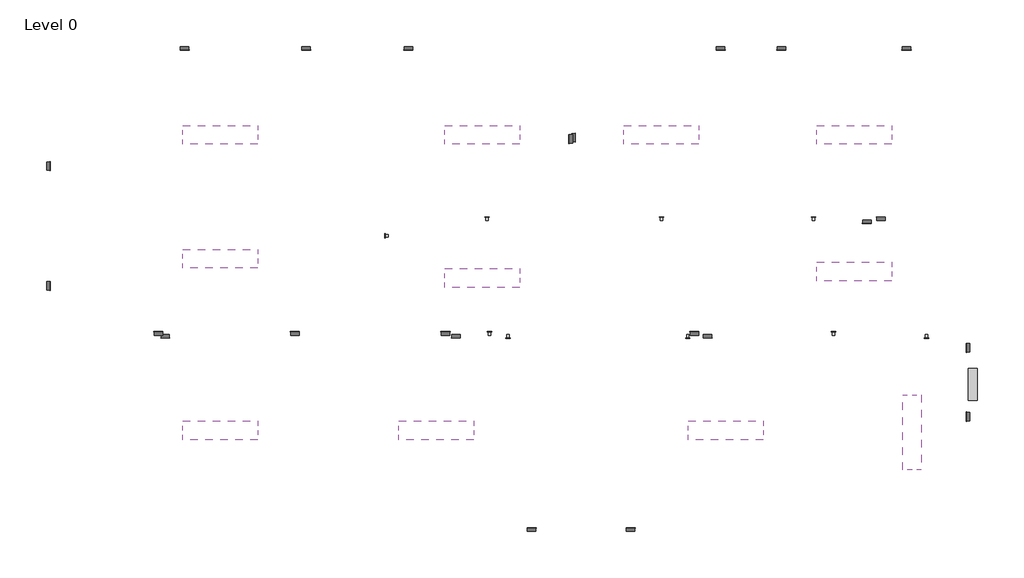
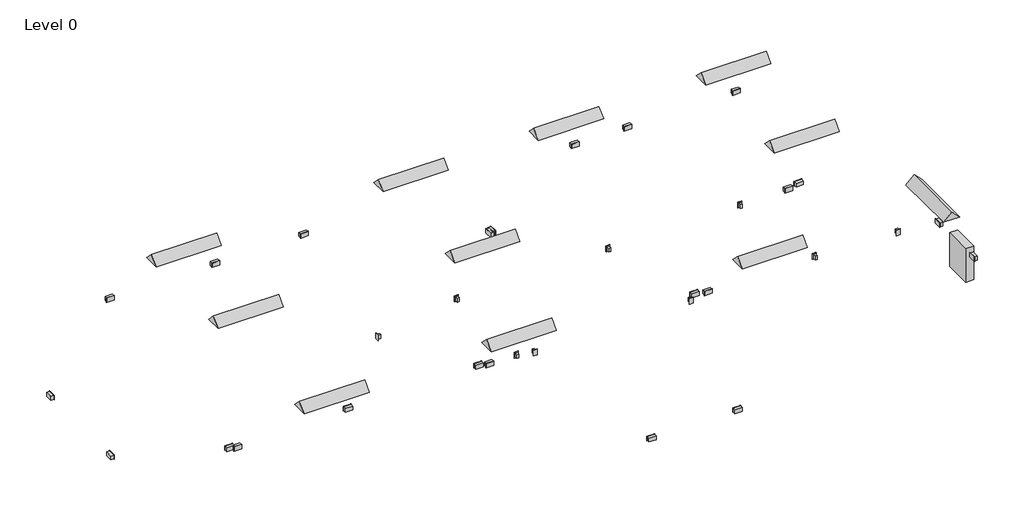
# One storey: 24 proxies, 11 light fixtures, 9 switching devices.
"""IFC4 building model written with IfcOpenShell, lengths in millimetres."""

import ifcopenshell
import ifcopenshell.guid

model = None  # the IFC model being written
_history = None  # IfcOwnerHistory: only IFC2X3 demands one
_inside = {}  # id of a spatial element -> (the spatial element, [elements in it])
_under = {}  # id of a project, library or spatial element -> (it, [spatial elements below it])
_declared = {}  # id of a project -> (the project, [libraries it declares])
_typed = {}  # id of a type object -> (the type object, [elements of that type])
_made_of = {}  # id of a material, layer set ... -> (it, [elements and type objects made of it])


def new_model(schema):
    """Start an empty IFC model of exactly this schema.

    Asked for "IFC4X3", IfcOpenShell would pick the latest addendum, in which some entities
    have other attributes; the version numbers below select the first issue.
    IFC2X3 requires an IfcOwnerHistory on every rooted entity: one is made here for all.
    """
    global model, _history
    if schema == "IFC4X3":
        model = ifcopenshell.file(schema_version=(4, 3, 0, 0))
    else:
        model = ifcopenshell.file(schema=schema)
    _inside.clear()
    _under.clear()
    _declared.clear()
    _typed.clear()
    _made_of.clear()
    _history = None
    if model.schema == "IFC2X3":
        org = make("IfcOrganization", Name="unknown")
        user = make(
            "IfcPersonAndOrganization",
            ThePerson=make("IfcPerson", FamilyName="unknown"),
            TheOrganization=org,
        )
        app = make(
            "IfcApplication",
            ApplicationDeveloper=org,
            Version="unknown",
            ApplicationFullName="unknown",
            ApplicationIdentifier="unknown",
        )
        _history = make(
            "IfcOwnerHistory",
            OwningUser=user,
            OwningApplication=app,
            ChangeAction="ADDED",
            CreationDate=0,
        )
    return model


def make(cls, **values):
    """One entity of the class cls with the attributes given. An attribute that is None is left unset."""
    return model.create_entity(
        cls, **{name: value for name, value in values.items() if value is not None}
    )


def rooted(cls, **values):
    """An entity with a GlobalId (a new one), such as an element, a storey or a relation."""
    return make(cls, GlobalId=ifcopenshell.guid.new(), OwnerHistory=_history, **values)


def si_unit(unit_type, name, prefix=None):
    """IfcSIUnit, for example si_unit("LENGTHUNIT", "METRE", prefix="MILLI")."""
    return make("IfcSIUnit", UnitType=unit_type, Prefix=prefix, Name=name)


def assignment(units):
    """IfcUnitAssignment: the units of a project."""
    return None if units is None else make("IfcUnitAssignment", Units=units)


def point(xyz):
    """IfcCartesianPoint."""
    return None if xyz is None else make("IfcCartesianPoint", Coordinates=xyz)


def direction(xyz):
    """IfcDirection."""
    return None if xyz is None else make("IfcDirection", DirectionRatios=xyz)


def frame(location, z_axis=None, x_axis=None):
    """IfcAxis2Placement3D, a coordinate frame: its origin and axes. An axis left out is left unset."""
    return make(
        "IfcAxis2Placement3D",
        Location=point(location),
        Axis=direction(z_axis),
        RefDirection=direction(x_axis),
    )


def origin():
    """The frame at (0, 0, 0) with its axes left unset."""
    return frame((0.0, 0.0, 0.0))


def origin_with_axes():
    """The frame at (0, 0, 0) with the z axis (0, 0, 1) and the x axis (1, 0, 0) written out."""
    return frame((0.0, 0.0, 0.0), z_axis=(0.0, 0.0, 1.0), x_axis=(1.0, 0.0, 0.0))


def place(relative_to, where):
    """IfcLocalPlacement: puts the frame where relative to a parent placement (None: the world)."""
    return make(
        "IfcLocalPlacement", PlacementRelTo=relative_to, RelativePlacement=where
    )


def context(
    kind, dimensions, precision=None, world=None, true_north=None, identifier=None
):
    """IfcGeometricRepresentationContext, for example the 3D "Model" context."""
    return make(
        "IfcGeometricRepresentationContext",
        ContextIdentifier=identifier,
        ContextType=kind,
        CoordinateSpaceDimension=dimensions,
        Precision=precision,
        WorldCoordinateSystem=world,
        TrueNorth=true_north,
    )


def project(units=None, contexts=None):
    """IfcProject with its units and contexts."""
    return rooted(
        "IfcProject",
        Name="project",
        RepresentationContexts=contexts,
        UnitsInContext=assignment(units),
    )


def spatial(cls, under=None, at=None, **own):
    """A site, building, storey or space (cls), placed at a placement, below another one or the project."""
    s = rooted(cls, ObjectPlacement=at, **own)
    if under is not None:
        _under.setdefault(under.id(), (under, []))[1].append(s)
    return s


def polyline(points):
    """IfcPolyline through the points."""
    return make("IfcPolyline", Points=[point(p) for p in points])


def outline(outer, holes=None, kind="AREA"):
    """IfcArbitraryClosedProfileDef: a profile drawn as a closed curve; with holes, ...WithVoids."""
    if holes is None:
        return make("IfcArbitraryClosedProfileDef", ProfileType=kind, OuterCurve=outer)
    return make(
        "IfcArbitraryProfileDefWithVoids",
        ProfileType=kind,
        OuterCurve=outer,
        InnerCurves=holes,
    )


def extrude(swept, where, along, depth):
    """IfcExtrudedAreaSolid: the profile swept, set in the frame where, extruded along a direction by depth."""
    return make(
        "IfcExtrudedAreaSolid",
        SweptArea=swept,
        Position=where,
        ExtrudedDirection=direction(along),
        Depth=depth,
    )


def shape(context_of_items, identifier, shape_type, items):
    """IfcShapeRepresentation: the items that make up one representation, for example the "Body"."""
    return make(
        "IfcShapeRepresentation",
        ContextOfItems=context_of_items,
        RepresentationIdentifier=identifier,
        RepresentationType=shape_type,
        Items=items,
    )


def source(mapping_origin, context_of_items, identifier, shape_type, items):
    """IfcRepresentationMap: a shape defined once, which mapped items show again and again."""
    return make(
        "IfcRepresentationMap",
        MappingOrigin=mapping_origin,
        MappedRepresentation=shape(context_of_items, identifier, shape_type, items),
    )


def transform(
    local_origin,
    x_axis=None,
    y_axis=None,
    z_axis=None,
    scale=None,
    scale2=None,
    scale3=None,
    uniform=True,
):
    """IfcCartesianTransformationOperator3D, or its non-uniform kind. x_axis, y_axis, z_axis: its Axis1, 2, 3."""
    if uniform:
        return make(
            "IfcCartesianTransformationOperator3D",
            Axis1=direction(x_axis),
            Axis2=direction(y_axis),
            LocalOrigin=point(local_origin),
            Scale=scale,
            Axis3=direction(z_axis),
        )
    return make(
        "IfcCartesianTransformationOperator3DnonUniform",
        Axis1=direction(x_axis),
        Axis2=direction(y_axis),
        LocalOrigin=point(local_origin),
        Scale=scale,
        Axis3=direction(z_axis),
        Scale2=scale2,
        Scale3=scale3,
    )


def mapped(mapping_source, mapping_target):
    """IfcMappedItem: shows the shape of a source again, moved by a transform."""
    return make(
        "IfcMappedItem", MappingSource=mapping_source, MappingTarget=mapping_target
    )


def made_of(thing, what):
    """Note that an element or type object is made of a material, layer set ...; save() writes the relation."""
    if what is not None:
        _made_of.setdefault(what.id(), (what, []))[1].append(thing)
    return thing


def element(
    cls,
    number,
    at=None,
    inside=None,
    cuts=None,
    type_object=None,
    material=None,
    context=None,
    identifier="Body",
    shape_type=None,
    held_by="IfcProductDefinitionShape",
    body=None,
    shapes=None,
    **own,
):
    """One element of the class cls, such as IfcWall. Its Tag is "e" and its number.

    at: its placement. inside: the storey or other place that contains it. cuts: it is an
    opening in that element (IfcRelVoidsElement). A single representation is given by context,
    identifier, shape_type and body (its items); several are given by shapes. held_by: the class
    of the entity that holds the representations. save() writes the other relations.
    """
    e = rooted(cls, Tag="e%d" % number, ObjectPlacement=at, **own)
    if body is not None:
        shapes = [shape(context, identifier, shape_type, body)]
    if shapes is not None:
        e.Representation = make(held_by, Representations=shapes)
    if inside is not None:
        _inside.setdefault(inside.id(), (inside, []))[1].append(e)
    if cuts is not None:
        rooted(
            "IfcRelVoidsElement", RelatingBuildingElement=cuts, RelatedOpeningElement=e
        )
    if type_object is not None:
        _typed.setdefault(type_object.id(), (type_object, []))[1].append(e)
    return made_of(e, material)


def aggregate(whole, parts):
    """IfcRelAggregates: a whole, such as a stair, and the parts it consists of."""
    return rooted("IfcRelAggregates", RelatingObject=whole, RelatedObjects=parts)


def save(model, path):
    """Write the relations noted so far, then the file.

    IfcRelAggregates (storeys below a building ...), IfcRelContainedInSpatialStructure (elements
    in a storey), IfcRelDefinesByType, IfcRelAssociatesMaterial and IfcRelDeclares: one each for
    every whole, place, type object, material and project.
    """
    for whole, parts in _under.values():
        aggregate(whole, parts)
    for where, things in _inside.values():
        rooted(
            "IfcRelContainedInSpatialStructure",
            RelatedElements=things,
            RelatingStructure=where,
        )
    for kind, things in _typed.values():
        rooted("IfcRelDefinesByType", RelatedObjects=things, RelatingType=kind)
    for what, things in _made_of.values():
        rooted("IfcRelAssociatesMaterial", RelatedObjects=things, RelatingMaterial=what)
    for by, libraries in _declared.values():
        rooted("IfcRelDeclares", RelatingContext=by, RelatedDefinitions=libraries)
    model.write(path)


def lighting_and_appliance_panelboard_400v_mlo_125_a_11cb7106(model_context):
    return source(origin(), model_context, "Body", "SweptSolid", [
        extrude(outline(polyline([(254.0, -660.4), (-254.0, -660.4), (-254.0, 0.0), (254.0, 0.0), (254.0, -660.4)])), frame((0.0, 0.0, -146.1), z_axis=(0.0, 0.0, 1.0), x_axis=(1.0, 0.0, 0.0)), (0.0, 0.0, 1.0), 146.1),
    ])


def twin_switched_socket_outlet_standard_0deee84c(model_context):
    return source(origin(), model_context, "Body", "SweptSolid", [
        extrude(outline(polyline([(67.5, 37.5), (67.5, -37.5), (-67.5, -37.5), (-67.5, 37.5), (67.5, 37.5)])), frame((0.0, 0.0, -53.975), z_axis=(0.0, 0.0, 1.0), x_axis=(1.0, 0.0, 0.0)), (0.0, 0.0, 1.0), 53.975),
        extrude(outline(polyline([(72.5, 42.5), (72.5, -42.5), (-72.5, -42.5), (-72.5, 42.5), (72.5, 42.5)])), origin_with_axes(), (0.0, 0.0, 1.0), 4.7625),
    ])


def plain_recessed_lighting_fixture_300x1200_230_e46e8774(model_context):
    return source(origin(), model_context, "Body", "SweptSolid", [
        extrude(outline(polyline([(-300.0, 0.0), (0.0, 0.0), (-150.0, -150.0), (-300.0, 0.0)])), frame((0.0, 0.0, 0.0), z_axis=(1.0, 0.0, 0.0), x_axis=(0.0, 1.0, 0.0)), (0.0, 0.0, 1.0), 1200.0),
    ])


def lighting_switches_one_way_switch_9cbd35ee(model_context):
    return source(origin(), model_context, "Body", "SweptSolid", [
        extrude(outline(polyline([(35.0, -114.0), (-35.0, -114.0), (-35.0, 0.0), (35.0, 0.0), (35.0, -114.0)])), origin_with_axes(), (0.0, 0.0, 1.0), 5.0),
        extrude(outline(polyline([(19.0, -95.0), (-19.0, -95.0), (-19.0, -19.0), (19.0, -19.0), (19.0, -95.0)])), frame((0.0, 0.0, -54.0), z_axis=(0.0, 0.0, 1.0), x_axis=(1.0, 0.0, 0.0)), (0.0, 0.0, 1.0), 54.0),
    ])


model = new_model("IFC4")

# Units and contexts
model_context = context("Model", 3, world=origin())
ifc_project = project(units=[si_unit("LENGTHUNIT", "METRE", prefix="MILLI")], contexts=[model_context])

# Site, building, storey
site = spatial("IfcSite", under=ifc_project)
building = spatial("IfcBuilding", under=site)
storey = spatial("IfcBuildingStorey", under=building, Name="Level 0", Elevation=0.0)

# Proxies
placement = place(None, origin())
lighting_and_appliance_panelboard_400v_mlo_125_a_shape = lighting_and_appliance_panelboard_400v_mlo_125_a_11cb7106(model_context)
element("IfcBuildingElementProxy", 1, Name="Lighting and Appliance Panelboard - 400V MLO : 125 A", ObjectType="Lighting and Appliance Panelboard - 400V MLO : 125 A", at=placement, inside=storey, context=model_context, shape_type="MappedRepresentation", body=[
    mapped(lighting_and_appliance_panelboard_400v_mlo_125_a_shape, transform((7508.0126521, -1234.1524125, 1200.0), x_axis=(0.0, 1.0, 0.0), y_axis=(0.0, 0.0, 1.0), z_axis=(1.0, 0.0, 0.0))),
])
twin_switched_socket_outlet_standard_shape = twin_switched_socket_outlet_standard_0deee84c(model_context)
element("IfcBuildingElementProxy", 2, Name="Twin Switched Socket Outlet : Standard", ObjectType="Twin Switched Socket Outlet : Standard", at=placement, inside=storey, context=model_context, shape_type="MappedRepresentation", body=[
    mapped(twin_switched_socket_outlet_standard_shape, transform((-7316.9873479, 344.9233542, 1200.0), x_axis=(0.0, 1.0, 0.0), y_axis=(0.0, 0.0, 1.0), z_axis=(1.0, 0.0, 0.0))),
])
element("IfcBuildingElementProxy", 3, Name="Twin Switched Socket Outlet : Standard", ObjectType="Twin Switched Socket Outlet : Standard", at=placement, inside=storey, context=model_context, shape_type="MappedRepresentation", body=[
    mapped(twin_switched_socket_outlet_standard_shape, transform((-7316.9873479, 2259.7123437, 1200.0), x_axis=(0.0, 1.0, 0.0), y_axis=(0.0, 0.0, 1.0), z_axis=(1.0, 0.0, 0.0))),
])
element("IfcBuildingElementProxy", 4, Name="Twin Switched Socket Outlet : Standard", ObjectType="Twin Switched Socket Outlet : Standard", at=placement, inside=storey, context=model_context, shape_type="MappedRepresentation", body=[
    mapped(twin_switched_socket_outlet_standard_shape, transform((-5162.5594983, 4119.0685046, 1200.0), x_axis=(1.0, 0.0, 0.0), y_axis=(0.0, 0.0, 1.0), z_axis=(0.0, -1.0, 0.0))),
])
element("IfcBuildingElementProxy", 5, Name="Twin Switched Socket Outlet : Standard", ObjectType="Twin Switched Socket Outlet : Standard", at=placement, inside=storey, context=model_context, shape_type="MappedRepresentation", body=[
    mapped(twin_switched_socket_outlet_standard_shape, transform((-3222.2399889, 4119.0685046, 1200.0), x_axis=(1.0, 0.0, 0.0), y_axis=(0.0, 0.0, 1.0), z_axis=(0.0, -1.0, 0.0))),
])
element("IfcBuildingElementProxy", 6, Name="Twin Switched Socket Outlet : Standard", ObjectType="Twin Switched Socket Outlet : Standard", at=placement, inside=storey, context=model_context, shape_type="MappedRepresentation", body=[
    mapped(twin_switched_socket_outlet_standard_shape, transform((-5583.813076, -393.4314954, 1200.0), x_axis=(-1.0, 0.0, 0.0), y_axis=(0.0, 0.0, 1.0), z_axis=(0.0, 1.0, 0.0))),
])
element("IfcBuildingElementProxy", 7, Name="Twin Switched Socket Outlet : Standard", ObjectType="Twin Switched Socket Outlet : Standard", at=placement, inside=storey, context=model_context, shape_type="MappedRepresentation", body=[
    mapped(twin_switched_socket_outlet_standard_shape, transform((-3400.9536279, -393.4314954, 1200.0), x_axis=(-1.0, 0.0, 0.0), y_axis=(0.0, 0.0, 1.0), z_axis=(0.0, 1.0, 0.0))),
])
element("IfcBuildingElementProxy", 8, Name="Twin Switched Socket Outlet : Standard", ObjectType="Twin Switched Socket Outlet : Standard", at=placement, inside=storey, context=model_context, shape_type="MappedRepresentation", body=[
    mapped(twin_switched_socket_outlet_standard_shape, transform((-1588.2867179, 4119.0685046, 1200.0), x_axis=(1.0, 0.0, 0.0), y_axis=(0.0, 0.0, 1.0), z_axis=(0.0, -1.0, 0.0))),
])
element("IfcBuildingElementProxy", 9, Name="Twin Switched Socket Outlet : Standard", ObjectType="Twin Switched Socket Outlet : Standard", at=placement, inside=storey, context=model_context, shape_type="MappedRepresentation", body=[
    mapped(twin_switched_socket_outlet_standard_shape, transform((983.0126521, 2693.7311813, 1200.0), x_axis=(0.0, -1.0, 0.0), y_axis=(0.0, 0.0, 1.0), z_axis=(-1.0, 0.0, 0.0))),
])
element("IfcBuildingElementProxy", 10, Name="Twin Switched Socket Outlet : Standard", ObjectType="Twin Switched Socket Outlet : Standard", at=placement, inside=storey, context=model_context, shape_type="MappedRepresentation", body=[
    mapped(twin_switched_socket_outlet_standard_shape, transform((1078.0126521, 2715.1886491, 1200.0), x_axis=(0.0, 1.0, 0.0), y_axis=(0.0, 0.0, 1.0), z_axis=(1.0, 0.0, 0.0))),
])
element("IfcBuildingElementProxy", 11, Name="Twin Switched Socket Outlet : Standard", ObjectType="Twin Switched Socket Outlet : Standard", at=placement, inside=storey, context=model_context, shape_type="MappedRepresentation", body=[
    mapped(twin_switched_socket_outlet_standard_shape, transform((3403.438978, 4119.0685046, 1200.0), x_axis=(1.0, 0.0, 0.0), y_axis=(0.0, 0.0, 1.0), z_axis=(0.0, -1.0, 0.0))),
])
element("IfcBuildingElementProxy", 12, Name="Twin Switched Socket Outlet : Standard", ObjectType="Twin Switched Socket Outlet : Standard", at=placement, inside=storey, context=model_context, shape_type="MappedRepresentation", body=[
    mapped(twin_switched_socket_outlet_standard_shape, transform((4374.4672873, 4119.0685046, 1200.0), x_axis=(1.0, 0.0, 0.0), y_axis=(0.0, 0.0, 1.0), z_axis=(0.0, -1.0, 0.0))),
])
element("IfcBuildingElementProxy", 13, Name="Twin Switched Socket Outlet : Standard", ObjectType="Twin Switched Socket Outlet : Standard", at=placement, inside=storey, context=model_context, shape_type="MappedRepresentation", body=[
    mapped(twin_switched_socket_outlet_standard_shape, transform((6373.6432184, 4119.0685046, 1200.0), x_axis=(1.0, 0.0, 0.0), y_axis=(0.0, 0.0, 1.0), z_axis=(0.0, -1.0, 0.0))),
])
element("IfcBuildingElementProxy", 14, Name="Twin Switched Socket Outlet : Standard", ObjectType="Twin Switched Socket Outlet : Standard", at=placement, inside=storey, context=model_context, shape_type="MappedRepresentation", body=[
    mapped(twin_switched_socket_outlet_standard_shape, transform((5963.2885588, 1441.5685046, 1200.0), x_axis=(-1.0, 0.0, 0.0), y_axis=(0.0, 0.0, 1.0), z_axis=(0.0, 1.0, 0.0))),
])
element("IfcBuildingElementProxy", 15, Name="Twin Switched Socket Outlet : Standard", ObjectType="Twin Switched Socket Outlet : Standard", at=placement, inside=storey, context=model_context, shape_type="MappedRepresentation", body=[
    mapped(twin_switched_socket_outlet_standard_shape, transform((5739.8085419, 1346.5685046, 1200.0), x_axis=(1.0, 0.0, 0.0), y_axis=(0.0, 0.0, 1.0), z_axis=(0.0, -1.0, 0.0))),
])
element("IfcBuildingElementProxy", 16, Name="Twin Switched Socket Outlet : Standard", ObjectType="Twin Switched Socket Outlet : Standard", at=placement, inside=storey, context=model_context, shape_type="MappedRepresentation", body=[
    mapped(twin_switched_socket_outlet_standard_shape, transform((2982.6225335, -393.4314954, 1200.0), x_axis=(-1.0, 0.0, 0.0), y_axis=(0.0, 0.0, 1.0), z_axis=(0.0, 1.0, 0.0))),
])
element("IfcBuildingElementProxy", 17, Name="Twin Switched Socket Outlet : Standard", ObjectType="Twin Switched Socket Outlet : Standard", at=placement, inside=storey, context=model_context, shape_type="MappedRepresentation", body=[
    mapped(twin_switched_socket_outlet_standard_shape, transform((3194.2813186, -488.4314954, 1200.0), x_axis=(1.0, 0.0, 0.0), y_axis=(0.0, 0.0, 1.0), z_axis=(0.0, -1.0, 0.0))),
])
element("IfcBuildingElementProxy", 18, Name="Twin Switched Socket Outlet : Standard", ObjectType="Twin Switched Socket Outlet : Standard", at=placement, inside=storey, context=model_context, shape_type="MappedRepresentation", body=[
    mapped(twin_switched_socket_outlet_standard_shape, transform((-994.162296, -393.4314954, 1200.0), x_axis=(-1.0, 0.0, 0.0), y_axis=(0.0, 0.0, 1.0), z_axis=(0.0, 1.0, 0.0))),
])
element("IfcBuildingElementProxy", 19, Name="Twin Switched Socket Outlet : Standard", ObjectType="Twin Switched Socket Outlet : Standard", at=placement, inside=storey, context=model_context, shape_type="MappedRepresentation", body=[
    mapped(twin_switched_socket_outlet_standard_shape, transform((-829.1509493, -488.4314954, 1200.0), x_axis=(1.0, 0.0, 0.0), y_axis=(0.0, 0.0, 1.0), z_axis=(0.0, -1.0, 0.0))),
])
element("IfcBuildingElementProxy", 20, Name="Twin Switched Socket Outlet : Standard", ObjectType="Twin Switched Socket Outlet : Standard", at=placement, inside=storey, context=model_context, shape_type="MappedRepresentation", body=[
    mapped(twin_switched_socket_outlet_standard_shape, transform((-5473.8620935, -488.4314954, 1200.0), x_axis=(1.0, 0.0, 0.0), y_axis=(0.0, 0.0, 1.0), z_axis=(0.0, -1.0, 0.0))),
])
element("IfcBuildingElementProxy", 21, Name="Twin Switched Socket Outlet : Standard", ObjectType="Twin Switched Socket Outlet : Standard", at=placement, inside=storey, context=model_context, shape_type="MappedRepresentation", body=[
    mapped(twin_switched_socket_outlet_standard_shape, transform((382.2243218, -3530.9314954, 1200.0), x_axis=(-1.0, 0.0, 0.0), y_axis=(0.0, 0.0, 1.0), z_axis=(0.0, 1.0, 0.0))),
])
element("IfcBuildingElementProxy", 22, Name="Twin Switched Socket Outlet : Standard", ObjectType="Twin Switched Socket Outlet : Standard", at=placement, inside=storey, context=model_context, shape_type="MappedRepresentation", body=[
    mapped(twin_switched_socket_outlet_standard_shape, transform((1965.1165531, -3530.9314954, 1200.0), x_axis=(-1.0, 0.0, 0.0), y_axis=(0.0, 0.0, 1.0), z_axis=(0.0, 1.0, 0.0))),
])
element("IfcBuildingElementProxy", 23, Name="Twin Switched Socket Outlet : Standard", ObjectType="Twin Switched Socket Outlet : Standard", at=placement, inside=storey, context=model_context, shape_type="MappedRepresentation", body=[
    mapped(twin_switched_socket_outlet_standard_shape, transform((7333.0126521, -1748.4570447, 1200.0), x_axis=(0.0, -1.0, 0.0), y_axis=(0.0, 0.0, 1.0), z_axis=(-1.0, 0.0, 0.0))),
])
element("IfcBuildingElementProxy", 24, Name="Twin Switched Socket Outlet : Standard", ObjectType="Twin Switched Socket Outlet : Standard", at=placement, inside=storey, context=model_context, shape_type="MappedRepresentation", body=[
    mapped(twin_switched_socket_outlet_standard_shape, transform((7333.0126521, -648.4570447, 1200.0), x_axis=(0.0, -1.0, 0.0), y_axis=(0.0, 0.0, 1.0), z_axis=(-1.0, 0.0, 0.0))),
])

# Light fixtures
plain_recessed_lighting_fixture_300x1200_230_shape = plain_recessed_lighting_fixture_300x1200_230_e46e8774(model_context)
element("IfcLightFixture", 25, ObjectType="Plain Recessed Lighting Fixture : 300x1200 - 230", at=placement, inside=storey, context=model_context, shape_type="MappedRepresentation", body=[
    mapped(plain_recessed_lighting_fixture_300x1200_230_shape, transform((-5192.3638129, 2609.1348514, 2750.0), x_axis=(1.0, 0.0, 0.0), y_axis=(0.0, -1.0, 0.0), z_axis=(0.0, 0.0, -1.0))),
])
element("IfcLightFixture", 26, ObjectType="Plain Recessed Lighting Fixture : 300x1200 - 230", at=placement, inside=storey, context=model_context, shape_type="MappedRepresentation", body=[
    mapped(plain_recessed_lighting_fixture_300x1200_230_shape, transform((-5192.3638129, 627.3282473, 2750.0), x_axis=(1.0, 0.0, 0.0), y_axis=(0.0, -1.0, 0.0), z_axis=(0.0, 0.0, -1.0))),
])
element("IfcLightFixture", 27, ObjectType="Plain Recessed Lighting Fixture : 300x1200 - 230", at=placement, inside=storey, context=model_context, shape_type="MappedRepresentation", body=[
    mapped(plain_recessed_lighting_fixture_300x1200_230_shape, transform((-1008.5498708, 2609.1348514, 2750.0), x_axis=(1.0, 0.0, 0.0), y_axis=(0.0, -1.0, 0.0), z_axis=(0.0, 0.0, -1.0))),
])
element("IfcLightFixture", 28, ObjectType="Plain Recessed Lighting Fixture : 300x1200 - 230", at=placement, inside=storey, context=model_context, shape_type="MappedRepresentation", body=[
    mapped(plain_recessed_lighting_fixture_300x1200_230_shape, transform((1854.0596685, 2609.1348514, 2750.0), x_axis=(1.0, 0.0, 0.0), y_axis=(0.0, -1.0, 0.0), z_axis=(0.0, 0.0, -1.0))),
])
element("IfcLightFixture", 29, ObjectType="Plain Recessed Lighting Fixture : 300x1200 - 230", at=placement, inside=storey, context=model_context, shape_type="MappedRepresentation", body=[
    mapped(plain_recessed_lighting_fixture_300x1200_230_shape, transform((4936.8699416, 2609.1348514, 2750.0), x_axis=(1.0, 0.0, 0.0), y_axis=(0.0, -1.0, 0.0), z_axis=(0.0, 0.0, -1.0))),
])
element("IfcLightFixture", 30, ObjectType="Plain Recessed Lighting Fixture : 300x1200 - 230", at=placement, inside=storey, context=model_context, shape_type="MappedRepresentation", body=[
    mapped(plain_recessed_lighting_fixture_300x1200_230_shape, transform((-1008.5498708, 319.04722, 2750.0), x_axis=(1.0, 0.0, 0.0), y_axis=(0.0, -1.0, 0.0), z_axis=(0.0, 0.0, -1.0))),
])
element("IfcLightFixture", 31, ObjectType="Plain Recessed Lighting Fixture : 300x1200 - 230", at=placement, inside=storey, context=model_context, shape_type="MappedRepresentation", body=[
    mapped(plain_recessed_lighting_fixture_300x1200_230_shape, transform((4936.8699416, 421.8075624, 2750.0), x_axis=(1.0, 0.0, 0.0), y_axis=(0.0, -1.0, 0.0), z_axis=(0.0, 0.0, -1.0))),
])
element("IfcLightFixture", 32, ObjectType="Plain Recessed Lighting Fixture : 300x1200 - 230", at=placement, inside=storey, context=model_context, shape_type="MappedRepresentation", body=[
    mapped(plain_recessed_lighting_fixture_300x1200_230_shape, transform((-5192.3638129, -2117.8409007, 2750.0), x_axis=(1.0, 0.0, 0.0), y_axis=(0.0, -1.0, 0.0), z_axis=(0.0, 0.0, -1.0))),
])
element("IfcLightFixture", 33, ObjectType="Plain Recessed Lighting Fixture : 300x1200 - 230", at=placement, inside=storey, context=model_context, shape_type="MappedRepresentation", body=[
    mapped(plain_recessed_lighting_fixture_300x1200_230_shape, transform((-1742.5523168, -2117.8409007, 2750.0), x_axis=(1.0, 0.0, 0.0), y_axis=(0.0, -1.0, 0.0), z_axis=(0.0, 0.0, -1.0))),
])
element("IfcLightFixture", 34, ObjectType="Plain Recessed Lighting Fixture : 300x1200 - 230", at=placement, inside=storey, context=model_context, shape_type="MappedRepresentation", body=[
    mapped(plain_recessed_lighting_fixture_300x1200_230_shape, transform((2881.6630929, -2117.8409007, 2750.0), x_axis=(1.0, 0.0, 0.0), y_axis=(0.0, -1.0, 0.0), z_axis=(0.0, 0.0, -1.0))),
])
element("IfcLightFixture", 35, ObjectType="Plain Recessed Lighting Fixture : 300x1200 - 230", at=placement, inside=storey, context=model_context, shape_type="MappedRepresentation", body=[
    mapped(plain_recessed_lighting_fixture_300x1200_230_shape, transform((6313.0126521, -1398.4314954, 2750.0), x_axis=(0.0, -1.0, 0.0), y_axis=(-1.0, 0.0, 0.0), z_axis=(0.0, 0.0, -1.0))),
])

# Switching devices
lighting_switches_one_way_switch_shape = lighting_switches_one_way_switch_9cbd35ee(model_context)
element("IfcSwitchingDevice", 36, ObjectType="Lighting Switches : One Way Switch", at=placement, inside=storey, context=model_context, shape_type="MappedRepresentation", body=[
    mapped(lighting_switches_one_way_switch_shape, transform((-1959.4873479, 1147.5444135, 1200.0), x_axis=(0.0, -1.0, 0.0), y_axis=(0.0, 0.0, 1.0), z_axis=(-1.0, 0.0, 0.0))),
])
element("IfcSwitchingDevice", 37, ObjectType="Lighting Switches : One Way Switch", at=placement, inside=storey, context=model_context, shape_type="MappedRepresentation", body=[
    mapped(lighting_switches_one_way_switch_shape, transform((-329.0865035, 1441.5685046, 1200.0), x_axis=(-1.0, 0.0, 0.0), y_axis=(0.0, 0.0, 1.0), z_axis=(0.0, 1.0, 0.0))),
])
element("IfcSwitchingDevice", 38, ObjectType="Lighting Switches : One Way Switch", at=placement, inside=storey, context=model_context, shape_type="MappedRepresentation", body=[
    mapped(lighting_switches_one_way_switch_shape, transform((2460.4485587, 1441.5685046, 1200.0), x_axis=(-1.0, 0.0, 0.0), y_axis=(0.0, 0.0, 1.0), z_axis=(0.0, 1.0, 0.0))),
])
element("IfcSwitchingDevice", 39, ObjectType="Lighting Switches : One Way Switch", at=placement, inside=storey, context=model_context, shape_type="MappedRepresentation", body=[
    mapped(lighting_switches_one_way_switch_shape, transform((4887.9777352, 1441.5685046, 1200.0), x_axis=(-1.0, 0.0, 0.0), y_axis=(0.0, 0.0, 1.0), z_axis=(0.0, 1.0, 0.0))),
])
element("IfcSwitchingDevice", 40, ObjectType="Lighting Switches : One Way Switch", at=placement, inside=storey, context=model_context, shape_type="MappedRepresentation", body=[
    mapped(lighting_switches_one_way_switch_shape, transform((6696.1000384, -488.4314954, 1200.0), x_axis=(1.0, 0.0, 0.0), y_axis=(0.0, 0.0, 1.0), z_axis=(0.0, -1.0, 0.0))),
])
element("IfcSwitchingDevice", 41, ObjectType="Lighting Switches : One Way Switch", at=placement, inside=storey, context=model_context, shape_type="MappedRepresentation", body=[
    mapped(lighting_switches_one_way_switch_shape, transform((2877.6222854, -488.4314954, 1200.0), x_axis=(1.0, 0.0, 0.0), y_axis=(0.0, 0.0, 1.0), z_axis=(0.0, -1.0, 0.0))),
])
element("IfcSwitchingDevice", 42, ObjectType="Lighting Switches : One Way Switch", at=placement, inside=storey, context=model_context, shape_type="MappedRepresentation", body=[
    mapped(lighting_switches_one_way_switch_shape, transform((2.6637447, -488.4314954, 1200.0), x_axis=(1.0, 0.0, 0.0), y_axis=(0.0, 0.0, 1.0), z_axis=(0.0, -1.0, 0.0))),
])
element("IfcSwitchingDevice", 43, ObjectType="Lighting Switches : Two Way Switch", at=placement, inside=storey, context=model_context, shape_type="MappedRepresentation", body=[
    mapped(lighting_switches_one_way_switch_shape, transform((-288.5833294, -393.4314954, 1200.0), x_axis=(-1.0, 0.0, 0.0), y_axis=(0.0, 0.0, 1.0), z_axis=(0.0, 1.0, 0.0))),
])
element("IfcSwitchingDevice", 44, ObjectType="Lighting Switches : Two Way Switch", at=placement, inside=storey, context=model_context, shape_type="MappedRepresentation", body=[
    mapped(lighting_switches_one_way_switch_shape, transform((5205.3500117, -393.4314954, 1200.0), x_axis=(-1.0, 0.0, 0.0), y_axis=(0.0, 0.0, 1.0), z_axis=(0.0, 1.0, 0.0))),
])

save(model, "model.ifc")

# Revit data of these elements
# Project information
#   Project Issue Date = "Oct 2020"
#   Project Status = "Project Status"
#   Client Name = "Owner"
#   Project Address = "Enter address here"
#   Project Name = "Revit MEP 01"
#   Project Number = "RMEP01"
# Type "Lighting and Appliance Panelboard - 400V MLO : 125 A"
#   built-in parameter 1140081 [instance default] = "Recessed"
#   built-in parameter 1140083 [instance default] = "Type 1"
#   Width = 508 mm
#   built-in parameter 1140082 [instance default] = 100 (stored number, unit not read)
#   built-in parameter 1140140 [instance default] = 1 (stored number, unit not read)
#   Height [instance default] = 660.4 mm
#   Depth = 146.1 mm
#   Default Elevation = 1200 mm
#   42 Circuit Height = 1117.6 mm
#   30 Circuit Height = 965.2 mm
#   18 Circuit Height = 660.4 mm
#   12 Circuit Height = 660.4 mm
#   built-in parameter 1140142 [instance default] = -1
#   built-in parameter 1140079 [instance default] = 12
#   built-in parameter 1155100 [instance default] = -1
#   Load Classification = Other
#   built-in parameter 1140087 [instance default] = element -7000014
# Type "Twin Switched Socket Outlet : Standard"
#   Label = "2"
#   Switch Voltage = 230 V
#   Load = 180 VA
#   Default Elevation = 1200 mm
#   Load Classification = Socket
#   Assembly Code = ""
# Type "Plain Recessed Lighting Fixture : 300x1200 - 230"
#   Photometric Web File = "1x42A12.ies"
#   Width = 300 mm
#   Wattage = 64 W
#   built-in parameter 1150110 = 1 (stored number, unit not read)
#   built-in parameter 1150109 = 1 (stored number, unit not read)
#   built-in parameter 1150113 = 1 (stored number, unit not read)
#   Tilt Angle = -90.00°
#   Lumens = 5699.84 lm
#   built-in parameter 1114217 = 0.88 (stored number, unit not read)
#   built-in parameter 1150115 = 1 (stored number, unit not read)
#   built-in parameter 1150105 = 453.579 (stored number, unit not read)
#   Length = 1200 mm
#   built-in parameter 1150112 = 1 (stored number, unit not read)
#   built-in parameter 1150114 = 1 (stored number, unit not read)
#   built-in parameter 1150107 = 4230 (stored number, unit not read)
#   built-in parameter 1150106 = 4.53579 (stored number, unit not read)
#   Emit from Rectangle Width = 300 mm
#   Emit from Rectangle Length = 1200 mm
#   built-in parameter 1150104 = 8.27394 (stored number, unit not read)
#   Depth = 150 mm
#   Default Elevation = 2000 mm
#   Ballast Voltage = 230 V
#   built-in parameter 1114218 = 0.88 (stored number, unit not read)
#   built-in parameter 1150133 = 10 (stored number, unit not read)
#   Apparent Load = 64 VA
#   built-in parameter 1150134 = 8
#   built-in parameter 1150137 = 1
#   Color Filter = 16777215
#   built-in parameter 1140040 [instance default] = 1
#   Load Classification = Lighting - Dwelling Unit
#   Emit Shape Visible in Rendering = no
#   Dimming Lamp Color Temperature Shift = (empty or 0)
#   Assembly Code = ""
# Type "Lighting Switches : One Way Switch"
#   Label = ""
#   Width = 70 mm
#   Switch Voltage [instance default] = 230 V
#   Length = 114 mm
#   Height = 59 mm
#   Default Elevation = 1200 mm
#   Apparent Load = 0 VA
#   Visibility 7 = no
#   Visibility 6 = no
#   Visibility 5 = yes
#   Visibility 4 = no
#   Visibility 3 = no
#   Visibility 2 = no
#   Visibility 1 = no
#   Number of Poles = 1
#   Load Classification = Other
# Type "Lighting Switches : Two Way Switch"
#   Label = "2"
#   Width = 70 mm
#   Switch Voltage [instance default] = 230 V
#   Length = 114 mm
#   Height = 59 mm
#   Default Elevation = 1200 mm
#   Apparent Load = 0 VA
#   Visibility 7 = no
#   Visibility 6 = no
#   Visibility 5 = no
#   Visibility 4 = yes
#   Visibility 3 = no
#   Visibility 2 = no
#   Visibility 1 = no
#   Number of Poles = 1
#   Load Classification = Other
# Element 1 (IfcBuildingElementProxy, "Lighting and Appliance Panelboard - 400V MLO : 125 A")
#   built-in parameter 1140086 = "-"
#   built-in parameter 1140085 = "CRT"
#   Panel Name = "Main Panel"
#   Mark = "3"
#   built-in parameter 1140081 = "Recessed"
#   built-in parameter 1140083 = "Type 1"
#   built-in parameter 1140082 = 100 (stored number, unit not read)
#   built-in parameter 1140140 = 100 (stored number, unit not read)
#   Height = 660.4 mm
#   built-in parameter 1140142 = -1
#   built-in parameter 1140079 = 12
#   built-in parameter 1155100 = -1
#   built-in parameter 1140064 = 230/400 Wye
#   built-in parameter 1140087 = element -7000010
#   Phase Created = New Construction
# Element 2 (IfcBuildingElementProxy, "Twin Switched Socket Outlet : Standard")
#   Mark = "1"
#   Phase Created = New Construction
# Element 3 (IfcBuildingElementProxy, "Twin Switched Socket Outlet : Standard")
#   Mark = "2"
#   Phase Created = New Construction
# Element 4 (IfcBuildingElementProxy, "Twin Switched Socket Outlet : Standard")
#   Mark = "3"
#   Phase Created = New Construction
# Element 5 (IfcBuildingElementProxy, "Twin Switched Socket Outlet : Standard")
#   Mark = "4"
#   Phase Created = New Construction
# Element 6 (IfcBuildingElementProxy, "Twin Switched Socket Outlet : Standard")
#   Mark = "5"
#   Phase Created = New Construction
# Element 7 (IfcBuildingElementProxy, "Twin Switched Socket Outlet : Standard")
#   Mark = "6"
#   Phase Created = New Construction
# Element 8 (IfcBuildingElementProxy, "Twin Switched Socket Outlet : Standard")
#   Mark = "7"
#   Phase Created = New Construction
# Element 9 (IfcBuildingElementProxy, "Twin Switched Socket Outlet : Standard")
#   Mark = "8"
#   Phase Created = New Construction
# Element 10 (IfcBuildingElementProxy, "Twin Switched Socket Outlet : Standard")
#   Mark = "9"
#   Phase Created = New Construction
# Element 11 (IfcBuildingElementProxy, "Twin Switched Socket Outlet : Standard")
#   Mark = "10"
#   Phase Created = New Construction
# Element 12 (IfcBuildingElementProxy, "Twin Switched Socket Outlet : Standard")
#   Mark = "11"
#   Phase Created = New Construction
# Element 13 (IfcBuildingElementProxy, "Twin Switched Socket Outlet : Standard")
#   Mark = "12"
#   Phase Created = New Construction
# Element 14 (IfcBuildingElementProxy, "Twin Switched Socket Outlet : Standard")
#   Mark = "13"
#   Phase Created = New Construction
# Element 15 (IfcBuildingElementProxy, "Twin Switched Socket Outlet : Standard")
#   Mark = "14"
#   Phase Created = New Construction
# Element 16 (IfcBuildingElementProxy, "Twin Switched Socket Outlet : Standard")
#   Mark = "15"
#   Phase Created = New Construction
# Element 17 (IfcBuildingElementProxy, "Twin Switched Socket Outlet : Standard")
#   Mark = "16"
#   Phase Created = New Construction
# Element 18 (IfcBuildingElementProxy, "Twin Switched Socket Outlet : Standard")
#   Mark = "17"
#   Phase Created = New Construction
# Element 19 (IfcBuildingElementProxy, "Twin Switched Socket Outlet : Standard")
#   Mark = "18"
#   Phase Created = New Construction
# Element 20 (IfcBuildingElementProxy, "Twin Switched Socket Outlet : Standard")
#   Mark = "19"
#   Phase Created = New Construction
# Element 21 (IfcBuildingElementProxy, "Twin Switched Socket Outlet : Standard")
#   Mark = "20"
#   Phase Created = New Construction
# Element 22 (IfcBuildingElementProxy, "Twin Switched Socket Outlet : Standard")
#   Mark = "21"
#   Phase Created = New Construction
# Element 23 (IfcBuildingElementProxy, "Twin Switched Socket Outlet : Standard")
#   Mark = "22"
#   Phase Created = New Construction
# Element 24 (IfcBuildingElementProxy, "Twin Switched Socket Outlet : Standard")
#   Mark = "23"
#   Phase Created = New Construction
# Element 25 (IfcLightFixture, "Plain Recessed Lighting Fixture : 300x1200 - 230")
#   Mark = "3"
#   built-in parameter 1140040 = 1
#   Phase Created = New Construction
# Element 26 (IfcLightFixture, "Plain Recessed Lighting Fixture : 300x1200 - 230")
#   Mark = "4"
#   built-in parameter 1140040 = 1
#   Phase Created = New Construction
# Element 27 (IfcLightFixture, "Plain Recessed Lighting Fixture : 300x1200 - 230")
#   Mark = "5"
#   built-in parameter 1140040 = 1
#   Phase Created = New Construction
# Element 28 (IfcLightFixture, "Plain Recessed Lighting Fixture : 300x1200 - 230")
#   Mark = "6"
#   built-in parameter 1140040 = 1
#   Phase Created = New Construction
# Element 29 (IfcLightFixture, "Plain Recessed Lighting Fixture : 300x1200 - 230")
#   Mark = "7"
#   built-in parameter 1140040 = 1
#   Phase Created = New Construction
# Element 30 (IfcLightFixture, "Plain Recessed Lighting Fixture : 300x1200 - 230")
#   Mark = "8"
#   built-in parameter 1140040 = 1
#   Phase Created = New Construction
# Element 31 (IfcLightFixture, "Plain Recessed Lighting Fixture : 300x1200 - 230")
#   Mark = "9"
#   built-in parameter 1140040 = 1
#   Phase Created = New Construction
# Element 32 (IfcLightFixture, "Plain Recessed Lighting Fixture : 300x1200 - 230")
#   Mark = "10"
#   built-in parameter 1140040 = 1
#   Phase Created = New Construction
# Element 33 (IfcLightFixture, "Plain Recessed Lighting Fixture : 300x1200 - 230")
#   Mark = "11"
#   built-in parameter 1140040 = 1
#   Phase Created = New Construction
# Element 34 (IfcLightFixture, "Plain Recessed Lighting Fixture : 300x1200 - 230")
#   Mark = "12"
#   built-in parameter 1140040 = 1
#   Phase Created = New Construction
# Element 35 (IfcLightFixture, "Plain Recessed Lighting Fixture : 300x1200 - 230")
#   Mark = "13"
#   built-in parameter 1140040 = 1
#   Phase Created = New Construction
# Element 36 (IfcSwitchingDevice, "Lighting Switches : One Way Switch")
#   Switch ID = "MO-LS"
#   Mark = "1"
#   Switch Voltage = -0.092903 V
#   Phase Created = New Construction
# Element 37 (IfcSwitchingDevice, "Lighting Switches : One Way Switch")
#   Switch ID = "MR-1-LS"
#   Mark = "2"
#   Switch Voltage = -0.092903 V
#   Phase Created = New Construction
# Element 38 (IfcSwitchingDevice, "Lighting Switches : One Way Switch")
#   Switch ID = "MR-2-LS"
#   Mark = "3"
#   Switch Voltage = -0.092903 V
#   Phase Created = New Construction
# Element 39 (IfcSwitchingDevice, "Lighting Switches : One Way Switch")
#   Switch ID = "MGR-LS"
#   Mark = "4"
#   Switch Voltage = -0.092903 V
#   Phase Created = New Construction
# Element 40 (IfcSwitchingDevice, "Lighting Switches : One Way Switch")
#   Switch ID = "SERV-LS"
#   Mark = "5"
#   Switch Voltage = -0.092903 V
#   Phase Created = New Construction
# Element 41 (IfcSwitchingDevice, "Lighting Switches : One Way Switch")
#   Switch ID = "RA-LS"
#   Mark = "6"
#   Switch Voltage = -0.092903 V
#   Phase Created = New Construction
# Element 42 (IfcSwitchingDevice, "Lighting Switches : One Way Switch")
#   Switch ID = "PA-LS"
#   Mark = "7"
#   Switch Voltage = -0.092903 V
#   Phase Created = New Construction
# Element 43 (IfcSwitchingDevice, "Lighting Switches : Two Way Switch")
#   Switch ID = "COR-LS-A"
#   Mark = "8"
#   Switch Voltage = -0.092903 V
#   Phase Created = New Construction
# Element 44 (IfcSwitchingDevice, "Lighting Switches : Two Way Switch")
#   Switch ID = "COR-LS-B"
#   Mark = "9"
#   Switch Voltage = -0.092903 V
#   Phase Created = New Construction
